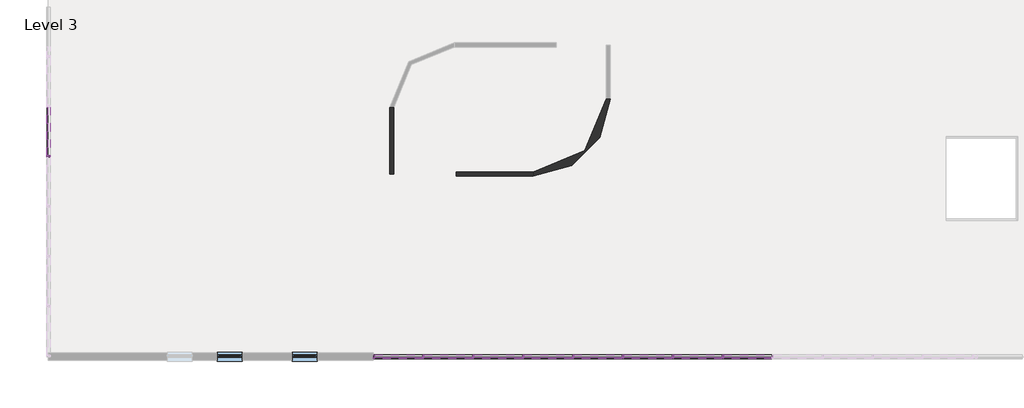
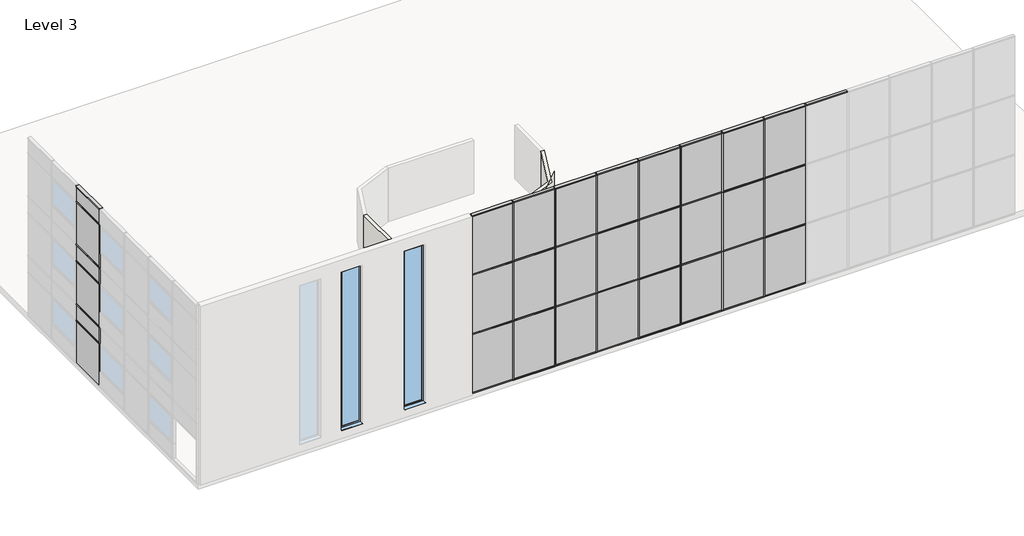
# One storey, part 2 of 5: 69 members, 30 plates, 3 walls, 2 windows.
# Revit data of these elements (continued)
# Type "Window - Variable : Standard" (continued)
#   Frame Depth = 0.060 m
#   Frame Height Bottom = 0.080 m
#   Frame Height Top = 0.080 m
#   Frame Width = 0.060 m
#   Height [instance default] = 1.010 m
#   Window Inset = 0.060 m
#   Window Width = 0.060 m
#   Instalation Depth [instance default] = 0.080 m
#   Width [instance default] = 1.010 m
#   Folding Wing [instance default] = no
#   Oppening Direction Vertical [instance default] = yes
#   Oppening Direction Visibility [instance default] = no
#   Casement [instance default] = yes
#   Frame [instance default] = none
#   Glas [instance default] = none
#   Window [instance default] = none
#   Windowsill Inside [instance default] = none
#   Windowsill Outside [instance default] = none
#   Wall Closure = (empty or 0)
#   Assembly Code = ""
# Elements 1, 2, 3, 4, 5, 6, 7, 8, 9, 10, 11, 12, 13, 14, 15, 16, 17, 18, 19, 20, 21, 22, 23, 24, 25, 26, 27, 28, 29, 30, 31, 32, 33, 34, 35, 36, 37, 38, 39, 40, 41, 42, 43, 44, 45, 46, 47, 48, 49, 50, 51, 52, 53, 54, 55, 56, 57, 58, 59, 60, 61, 62, 63, 64, 65, 66, 67, 68, 69 (IfcMember, "Rectangular Mullion : 50 x 150mm")
#   Phase Created = New Construction
#   Materials on its faces: "Metal - Aluminium"
# Elements 70, 71, 72, 73, 74, 75, 76, 77, 78, 79, 80, 81, 82, 83, 84, 85, 86, 87, 88, 89, 90, 91, 92, 93, 94, 95, 96, 97, 98, 99 (IfcPlate, "System Panel : Glazed")
#   Phase Created = New Construction
#   Materials on its faces: "Glass"
# Elements 100, 101 (IfcWall, "Interior - Blockwork 140")
#   Top Offset = -0.300 m
#   Base Offset = 0.000 m
#   wall height = 2.700 m
#   Phase Created = New Construction
#   Base Constraint = Level 3
#   Top Constraint = Level 4
#   Materials on its faces: "Default Wall", "Plasterboard"
# Element 102 (IfcWall, "Interior - Blockwork 140")
#   Top Offset = -0.300 m
#   Base Offset = 0.000 m
#   Unconnected Height = 4.000 m
#   wall height = 2.700 m
#   Phase Created = New Construction
#   Materials on its faces: "Default Wall", "Plasterboard"
# Element 103 (IfcWindow, "Window - Variable : Standard")
#   Mark = "9"
#   Width = 1.000 m
#   Rough Width = 1.000 m
#   Rough Height = 8.000 m
#   Instalation Depth = 0.080 m
#   Height = 8.000 m
#   Oppening Direction Visibility = no
#   Oppening Direction Vertical = yes
#   Folding Wing = no
#   Casement = yes
#   Windowsill Outside = none
#   Windowsill Inside = none
#   Window = none
#   Glas = none
#   Frame = none
#   Phase Created = New Construction
#   Materials on its faces: "Plastic - White", "Metal _ Aluminium", "Wood - Birch", "Glass"
# Element 104 (IfcWindow, "Window - Variable : Standard")
#   Mark = "10"
#   Width = 1.000 m
#   Rough Width = 1.000 m
#   Rough Height = 8.000 m
#   Instalation Depth = 0.080 m
#   Height = 8.000 m
#   Oppening Direction Visibility = no
#   Oppening Direction Vertical = yes
#   Folding Wing = no
#   Casement = yes
#   Windowsill Outside = none
#   Windowsill Inside = none
#   Window = none
#   Glas = none
#   Frame = none
#   Phase Created = New Construction
#   Materials on its faces: "Plastic - White", "Metal _ Aluminium", "Wood - Birch", "Glass"
# Materials
#   "Plasterboard": class "Drywall", colour RGB 249 249 249, transparency 0, Description = "Interior finish"
#   "Masonry - Concrete Block": class "Concrete", colour RGB 181 181 181, transparency 0
#   "Metal - Aluminium": class "Metal", colour RGB 247 247 247, transparency 0
#   "Glass": class "Glass", colour RGB 0 128 192, transparency 0.9
#   "Default Wall": class "Miscellaneous", colour RGB 128 128 128, transparency 0
#   "Plastic - White": class "Kunststoff", colour RGB 249 249 249, transparency 0
#   "Metal _ Aluminium": class "Metall", colour RGB 247 247 247, transparency 0
#   "Wood - Birch": class "Holz", colour RGB 213 164 103, transparency 0
